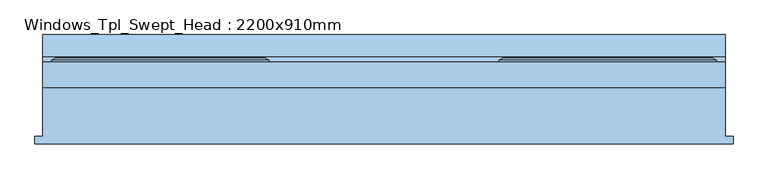
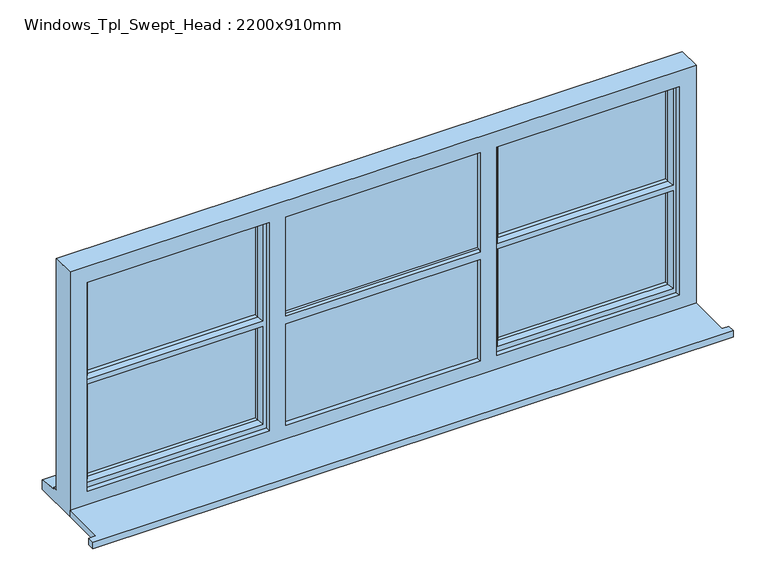
"""IFC4 building model written with IfcOpenShell, lengths in millimetres: window geometry, Windows_Tpl_Swept_Head : 2200x910mm."""

from ifc_helpers import new_model, si_unit, point, frame, frame_2d, origin, place, context, project, spatial, polyline, circle_curve, trimmed, segment, composite_curve, outline, extrude, faceted_brep, source, transform, mapped, element, save


def windows_tpl_swept_head_2200x910mm_9484ce63(model_context):
    return source(origin(), model_context, "Body", "SolidModel", [
        extrude(outline(polyline([(-1766.6666667, -161.5434322), (-1766.6666667, -136.5434322), (-1741.6666667, -136.5434322), (-1741.6666667, 20.4565678), (458.3333333, 20.4565678), (458.3333333, -136.5434322), (483.3333333, -136.5434322), (483.3333333, -161.5434322), (-1766.6666667, -161.5434322)])), frame((0.0, 0.0, 1200.0), z_axis=(0.0, 0.0, 1.0), x_axis=(1.0, 0.0, 0.0)), (0.0, 0.0, 1.0), 25.0),
        extrude(outline(composite_curve([segment(polyline([(2050.0, -300.0), (2050.0, -983.3333333), (1935.9532624, -983.3333333)]), True, "CONTINUOUS"), segment(trimmed(circle_curve(frame_2d((1325.0, -641.6666667)), 700.0), [point((1935.9532624, -983.3333333))], [point((1935.9532624, -300.0))], True, "CARTESIAN"), True, "CONTINUOUS"), segment(polyline([(1935.9532624, -300.0), (2050.0, -300.0)]), True, "CONTINUOUS")], self_intersect=False)), frame((0.0, 62.4565678, 0.0), z_axis=(0.0, 1.0, 0.0), x_axis=(0.0, 0.0, 1.0)), (0.0, 0.0, 1.0), 25.0),
        extrude(outline(composite_curve([segment(polyline([(2030.0, -220.0), (1957.8501446, -220.0)]), True, "CONTINUOUS"), segment(trimmed(circle_curve(frame_2d((1325.0, 79.1666667)), 700.0), [point((1957.8501446, -220.0))], [point((1957.8501446, 378.3333333))], True, "CARTESIAN"), True, "CONTINUOUS"), segment(polyline([(1957.8501446, 378.3333333), (2030.0, 378.3333333), (2030.0, -220.0)]), True, "CONTINUOUS")], self_intersect=False)), frame((0.0, 79.4565678, 0.0), z_axis=(0.0, 1.0, 0.0), x_axis=(0.0, 0.0, 1.0)), (0.0, 0.0, 1.0), 24.0),
        extrude(outline(composite_curve([segment(polyline([(2030.0, -1063.3333333), (2030.0, -1661.6666667), (1957.8501446, -1661.6666667)]), True, "CONTINUOUS"), segment(trimmed(circle_curve(frame_2d((1325.0, -1362.5)), 700.0), [point((1957.8501446, -1661.6666667))], [point((1957.8501446, -1063.3333333))], True, "CARTESIAN"), True, "CONTINUOUS"), segment(polyline([(1957.8501446, -1063.3333333), (2030.0, -1063.3333333)]), True, "CONTINUOUS")], self_intersect=False)), frame((0.0, 79.4565678, 0.0), z_axis=(0.0, 1.0, 0.0), x_axis=(0.0, 0.0, 1.0)), (0.0, 0.0, 1.0), 24.0),
        faceted_brep([(-270.0, 103.4565678, 2080.0), (-270.0, 109.2300705, 2080.0), (-270.0, 109.2300705, 1253.0), (-270.0, 103.4565678, 1253.0), (-260.0, 38.4565678, 2070.0), (-260.0, 103.4565678, 2070.0), (-260.0, 103.4565678, 1263.0), (-260.0, 38.4565678, 1263.0), (-220.0, 52.9494677, 2030.0), (-230.1480377, 38.4565678, 2040.1480377), (-230.1480377, 38.4565678, 1676.3519623), (-220.0, 52.9494677, 1686.5), (-230.1480377, 38.4565678, 1292.8519623), (-220.0, 52.9494677, 1303.0), (-220.0, 52.9494677, 1646.5), (-230.1480377, 38.4565678, 1656.6480377), (-220.0, 67.4565678, 2030.0), (-220.0, 67.4565678, 1686.5), (-220.0, 67.4565678, 1303.0), (-220.0, 67.4565678, 1646.5), (-230.0, 91.4565678, 1679.5), (-230.0, 91.4565678, 2040.0), (-230.0, 67.4565678, 2040.0), (-230.0, 67.4565678, 1679.5), (-230.0, 67.4565678, 1653.5), (-230.0, 67.4565678, 1293.0), (-230.0, 91.4565678, 1293.0), (-230.0, 91.4565678, 1653.5), (-220.0, 109.2300705, 2030.0), (-220.0, 91.4565678, 2030.0), (-220.0, 91.4565678, 1686.5), (-220.0, 109.2300705, 1686.5), (-220.0, 91.4565678, 1303.0), (-220.0, 109.2300705, 1303.0), (-220.0, 109.2300705, 1646.5), (-220.0, 91.4565678, 1646.5), (-237.4457548, 115.0035732, 2047.4457548), (-237.4457548, 115.0035732, 1669.0542452), (-237.4457548, 115.0035732, 1285.5542452), (-237.4457548, 115.0035732, 1663.9457548), (-259.2153903, 115.0035732, 2069.2153903), (-259.2153903, 115.0035732, 1263.7846097), (428.3333333, 109.2300705, 1253.0), (428.3333333, 103.4565678, 1253.0), (418.3333333, 103.4565678, 1263.0), (418.3333333, 38.4565678, 1263.0), (388.4813711, 38.4565678, 1292.8519623), (378.3333333, 52.9494677, 1303.0), (378.3333333, 67.4565678, 1303.0), (388.3333333, 67.4565678, 1293.0), (388.3333333, 91.4565678, 1293.0), (378.3333333, 91.4565678, 1303.0), (378.3333333, 109.2300705, 1303.0), (395.7790881, 115.0035732, 1285.5542452), (417.5487236, 115.0035732, 1263.7846097), (428.3333333, 109.2300705, 2080.0), (428.3333333, 103.4565678, 2080.0), (418.3333333, 103.4565678, 2070.0), (418.3333333, 38.4565678, 2070.0), (388.4813711, 38.4565678, 1656.6480377), (378.3333333, 52.9494677, 1646.5), (388.4813711, 38.4565678, 2040.1480377), (378.3333333, 52.9494677, 2030.0), (378.3333333, 52.9494677, 1686.5), (388.4813711, 38.4565678, 1676.3519623), (378.3333333, 67.4565678, 1646.5), (378.3333333, 67.4565678, 2030.0), (378.3333333, 67.4565678, 1686.5), (388.3333333, 91.4565678, 1653.5), (388.3333333, 67.4565678, 1653.5), (388.3333333, 67.4565678, 1679.5), (388.3333333, 67.4565678, 2040.0), (388.3333333, 91.4565678, 2040.0), (388.3333333, 91.4565678, 1679.5), (378.3333333, 91.4565678, 1646.5), (378.3333333, 109.2300705, 1646.5), (378.3333333, 91.4565678, 2030.0), (378.3333333, 109.2300705, 2030.0), (378.3333333, 109.2300705, 1686.5), (378.3333333, 91.4565678, 1686.5), (395.7790881, 115.0035732, 1663.9457548), (395.7790881, 115.0035732, 2047.4457548), (395.7790881, 115.0035732, 1669.0542452), (417.5487236, 115.0035732, 2069.2153903)], [[[0, 1, 2, 3]], [[4, 5, 6, 7]], [[8, 9, 10, 11]], [[12, 13, 14, 15]], [[16, 8, 11, 17]], [[13, 18, 19, 14]], [[20, 21, 22, 23]], [[24, 25, 26, 27]], [[28, 29, 30, 31]], [[32, 33, 34, 35]], [[36, 28, 31, 37]], [[33, 38, 39, 34]], [[2, 1, 40, 41]], [[3, 2, 42, 43]], [[7, 6, 44, 45]], [[13, 12, 46, 47]], [[18, 13, 47, 48]], [[26, 25, 49, 50]], [[33, 32, 51, 52]], [[38, 33, 52, 53]], [[2, 41, 54, 42]], [[43, 42, 55, 56]], [[45, 44, 57, 58]], [[47, 46, 59, 60]], [[61, 62, 63, 64]], [[48, 47, 60, 65]], [[62, 66, 67, 63]], [[68, 50, 49, 69]], [[70, 71, 72, 73]], [[52, 51, 74, 75]], [[76, 77, 78, 79]], [[53, 52, 75, 80]], [[77, 81, 82, 78]], [[42, 54, 83, 55]], [[1, 0, 56, 55]], [[0, 3, 43, 56], [6, 5, 57, 44]], [[5, 4, 58, 57]], [[4, 7, 45, 58], [46, 12, 15, 59], [61, 64, 10, 9]], [[9, 8, 62, 61]], [[8, 16, 66, 62]], [[49, 25, 24, 69], [18, 48, 65, 19]], [[22, 71, 70, 23], [66, 16, 17, 67]], [[22, 21, 72, 71]], [[26, 50, 68, 27], [32, 35, 74, 51]], [[72, 21, 20, 73], [76, 79, 30, 29]], [[29, 28, 77, 76]], [[28, 36, 81, 77]], [[41, 40, 83, 54], [36, 37, 82, 81], [38, 53, 80, 39]], [[40, 1, 55, 83]], [[82, 37, 31, 78]], [[30, 79, 78, 31]], [[73, 20, 23, 70]], [[11, 63, 67, 17]], [[10, 64, 63, 11]], [[59, 15, 14, 60]], [[60, 14, 19, 65]], [[27, 68, 69, 24]], [[74, 35, 34, 75]], [[39, 80, 75, 34]]]),
        faceted_brep([(-1013.3333333, 103.4565678, 2080.0), (-1013.3333333, 109.2300705, 2080.0), (-1711.6666667, 109.2300705, 2080.0), (-1711.6666667, 103.4565678, 2080.0), (-1023.3333333, 38.4565678, 2070.0), (-1023.3333333, 103.4565678, 2070.0), (-1701.6666667, 103.4565678, 2070.0), (-1701.6666667, 38.4565678, 2070.0), (-1063.3333333, 52.9494677, 2030.0), (-1053.1852956, 38.4565678, 2040.1480377), (-1671.8147044, 38.4565678, 2040.1480377), (-1661.6666667, 52.9494677, 2030.0), (-1661.6666667, 67.4565678, 2030.0), (-1063.3333333, 67.4565678, 2030.0), (-1053.3333333, 91.4565678, 2040.0), (-1053.3333333, 67.4565678, 2040.0), (-1671.6666667, 67.4565678, 2040.0), (-1671.6666667, 91.4565678, 2040.0), (-1063.3333333, 109.2300705, 2030.0), (-1063.3333333, 91.4565678, 2030.0), (-1661.6666667, 91.4565678, 2030.0), (-1661.6666667, 109.2300705, 2030.0), (-1679.1124215, 115.0035732, 2047.4457548), (-1045.8875785, 115.0035732, 2047.4457548), (-1024.117943, 115.0035732, 2069.2153903), (-1700.882057, 115.0035732, 2069.2153903), (-1711.6666667, 109.2300705, 1253.0), (-1711.6666667, 103.4565678, 1253.0), (-1701.6666667, 103.4565678, 1263.0), (-1701.6666667, 38.4565678, 1263.0), (-1671.8147044, 38.4565678, 1676.3519623), (-1661.6666667, 52.9494677, 1686.5), (-1671.8147044, 38.4565678, 1292.8519623), (-1661.6666667, 52.9494677, 1303.0), (-1661.6666667, 52.9494677, 1646.5), (-1671.8147044, 38.4565678, 1656.6480377), (-1661.6666667, 67.4565678, 1686.5), (-1661.6666667, 67.4565678, 1303.0), (-1661.6666667, 67.4565678, 1646.5), (-1671.6666667, 91.4565678, 1679.5), (-1671.6666667, 67.4565678, 1679.5), (-1671.6666667, 67.4565678, 1653.5), (-1671.6666667, 67.4565678, 1293.0), (-1671.6666667, 91.4565678, 1293.0), (-1671.6666667, 91.4565678, 1653.5), (-1661.6666667, 91.4565678, 1686.5), (-1661.6666667, 109.2300705, 1686.5), (-1661.6666667, 91.4565678, 1303.0), (-1661.6666667, 109.2300705, 1303.0), (-1661.6666667, 109.2300705, 1646.5), (-1661.6666667, 91.4565678, 1646.5), (-1679.1124215, 115.0035732, 1669.0542452), (-1679.1124215, 115.0035732, 1285.5542452), (-1679.1124215, 115.0035732, 1663.9457548), (-1700.882057, 115.0035732, 1263.7846097), (-1013.3333333, 109.2300705, 1253.0), (-1013.3333333, 103.4565678, 1253.0), (-1023.3333333, 103.4565678, 1263.0), (-1023.3333333, 38.4565678, 1263.0), (-1053.1852956, 38.4565678, 1676.3519623), (-1053.1852956, 38.4565678, 1656.6480377), (-1053.1852956, 38.4565678, 1292.8519623), (-1063.3333333, 52.9494677, 1303.0), (-1063.3333333, 67.4565678, 1303.0), (-1053.3333333, 67.4565678, 1679.5), (-1063.3333333, 67.4565678, 1686.5), (-1053.3333333, 67.4565678, 1293.0), (-1053.3333333, 67.4565678, 1653.5), (-1063.3333333, 67.4565678, 1646.5), (-1053.3333333, 91.4565678, 1293.0), (-1053.3333333, 91.4565678, 1679.5), (-1063.3333333, 91.4565678, 1686.5), (-1053.3333333, 91.4565678, 1653.5), (-1063.3333333, 91.4565678, 1646.5), (-1063.3333333, 91.4565678, 1303.0), (-1063.3333333, 109.2300705, 1303.0), (-1045.8875785, 115.0035732, 1285.5542452), (-1024.117943, 115.0035732, 1263.7846097), (-1045.8875785, 115.0035732, 1669.0542452), (-1045.8875785, 115.0035732, 1663.9457548), (-1063.3333333, 52.9494677, 1686.5), (-1063.3333333, 52.9494677, 1646.5), (-1063.3333333, 109.2300705, 1686.5), (-1063.3333333, 109.2300705, 1646.5)], [[[0, 1, 2, 3]], [[4, 5, 6, 7]], [[8, 9, 10, 11]], [[8, 11, 12, 13]], [[14, 15, 16, 17]], [[18, 19, 20, 21]], [[18, 21, 22, 23]], [[2, 1, 24, 25]], [[3, 2, 26, 27]], [[7, 6, 28, 29]], [[11, 10, 30, 31]], [[32, 33, 34, 35]], [[12, 11, 31, 36]], [[33, 37, 38, 34]], [[39, 17, 16, 40]], [[41, 42, 43, 44]], [[21, 20, 45, 46]], [[47, 48, 49, 50]], [[22, 21, 46, 51]], [[48, 52, 53, 49]], [[2, 25, 54, 26]], [[27, 26, 55, 56]], [[0, 3, 27, 56], [6, 5, 57, 28]], [[29, 28, 57, 58]], [[4, 7, 29, 58], [10, 9, 59, 30], [32, 35, 60, 61]], [[33, 32, 61, 62]], [[37, 33, 62, 63]], [[16, 15, 64, 40], [13, 12, 36, 65]], [[66, 42, 41, 67], [37, 63, 68, 38]], [[43, 42, 66, 69]], [[14, 17, 39, 70], [19, 71, 45, 20]], [[43, 69, 72, 44], [47, 50, 73, 74]], [[48, 47, 74, 75]], [[52, 48, 75, 76]], [[25, 24, 77, 54], [23, 22, 51, 78], [76, 79, 53, 52]], [[26, 54, 77, 55]], [[1, 0, 56, 55]], [[5, 4, 58, 57]], [[9, 8, 80, 59]], [[62, 61, 60, 81]], [[8, 13, 65, 80]], [[63, 62, 81, 68]], [[64, 15, 14, 70]], [[72, 69, 66, 67]], [[19, 18, 82, 71]], [[75, 74, 73, 83]], [[18, 23, 78, 82]], [[76, 75, 83, 79]], [[24, 1, 55, 77]], [[78, 51, 46, 82]], [[45, 71, 82, 46]], [[40, 64, 70, 39]], [[65, 36, 31, 80]], [[30, 59, 80, 31]], [[60, 35, 34, 81]], [[38, 68, 81, 34]], [[67, 41, 44, 72]], [[73, 50, 49, 83]], [[53, 79, 83, 49]]]),
        extrude(outline(polyline([(388.4813711, 67.4565678), (-230.0, 67.4565678), (-230.0, 91.4565678), (388.4813711, 91.4565678), (388.4813711, 67.4565678)])), frame((0.0, 0.0, 1293.0), z_axis=(0.0, 0.0, 1.0), x_axis=(1.0, 0.0, 0.0)), (0.0, 0.0, 1.0), 363.6480377),
        extrude(outline(polyline([(388.4813711, 67.4565678), (-230.0, 67.4565678), (-230.0, 91.4565678), (388.4813711, 91.4565678), (388.4813711, 67.4565678)])), frame((0.0, 0.0, 1676.3519623), z_axis=(0.0, 0.0, 1.0), x_axis=(1.0, 0.0, 0.0)), (0.0, 0.0, 1.0), 363.6480377),
        extrude(outline(polyline([(-993.3333333, 62.4565678), (-290.0, 62.4565678), (-290.0, 38.4565678), (-993.3333333, 38.4565678), (-993.3333333, 62.4565678)])), frame((0.0, 0.0, 1263.0), z_axis=(0.0, 0.0, 1.0), x_axis=(1.0, 0.0, 0.0)), (0.0, 0.0, 1.0), 390.5),
        extrude(outline(polyline([(-993.3333333, 62.4565678), (-290.0, 62.4565678), (-290.0, 38.4565678), (-993.3333333, 38.4565678), (-993.3333333, 62.4565678)])), frame((0.0, 0.0, 1679.5), z_axis=(0.0, 0.0, 1.0), x_axis=(1.0, 0.0, 0.0)), (0.0, 0.0, 1.0), 390.5),
        extrude(outline(polyline([(-1053.3333333, 67.4565678), (-1671.6666667, 67.4565678), (-1671.6666667, 91.4565678), (-1053.3333333, 91.4565678), (-1053.3333333, 67.4565678)])), frame((0.0, 0.0, 1676.3519623), z_axis=(0.0, 0.0, 1.0), x_axis=(1.0, 0.0, 0.0)), (0.0, 0.0, 1.0), 363.6480377),
        extrude(outline(polyline([(-1053.3333333, 67.4565678), (-1671.6666667, 67.4565678), (-1671.6666667, 91.4565678), (-1053.3333333, 91.4565678), (-1053.3333333, 67.4565678)])), frame((0.0, 0.0, 1293.0), z_axis=(0.0, 0.0, 1.0), x_axis=(1.0, 0.0, 0.0)), (0.0, 0.0, 1.0), 363.6480377),
        faceted_brep([(-983.3333333, 38.4565678, 2050.0), (-983.3333333, 20.4565678, 2050.0), (-983.3333333, 20.4565678, 1680.8390708), (-983.3333333, 28.5412125, 1686.5), (-983.3333333, 38.4565678, 1686.5), (-983.3333333, 20.4565678, 1275.0), (-983.3333333, 38.4565678, 1275.0), (-983.3333333, 38.4565678, 1646.5), (-983.3333333, 28.5412125, 1646.5), (-983.3333333, 20.4565678, 1652.1609292), (458.3333333, 20.4565678, 2110.0), (-1741.6666667, 20.4565678, 2110.0), (-1741.6666667, 20.4565678, 1200.0), (458.3333333, 20.4565678, 1200.0), (-1681.6666667, 20.4565678, 2050.0), (-1041.3333333, 20.4565678, 2050.0), (-1041.3333333, 20.4565678, 1275.0), (-1681.6666667, 20.4565678, 1275.0), (-242.0, 20.4565678, 2050.0), (398.3333333, 20.4565678, 2050.0), (398.3333333, 20.4565678, 1275.0), (-242.0, 20.4565678, 1275.0), (-300.0, 20.4565678, 2050.0), (-300.0, 20.4565678, 1680.8390708), (-300.0, 20.4565678, 1275.0), (-300.0, 20.4565678, 1652.1609292), (-1041.3333333, 38.4565678, 2050.0), (-1041.3333333, 38.4565678, 1275.0), (-1701.6666667, 38.4565678, 2070.0), (-1023.3333333, 38.4565678, 2070.0), (-1023.3333333, 38.4565678, 1263.0), (-1701.6666667, 38.4565678, 1263.0), (-1681.6666667, 38.4565678, 2050.0), (-1681.6666667, 38.4565678, 1275.0), (-993.3333333, 38.4565678, 2070.0), (-290.0, 38.4565678, 2070.0), (-290.0, 38.4565678, 1679.5), (-983.3333333, 38.4565678, 1679.5), (-983.3333333, 38.4565678, 1653.5), (-290.0, 38.4565678, 1653.5), (-290.0, 38.4565678, 1263.0), (-993.3333333, 38.4565678, 1263.0), (-300.0, 38.4565678, 2050.0), (-300.0, 38.4565678, 1686.5), (-300.0, 38.4565678, 1275.0), (-300.0, 38.4565678, 1646.5), (-260.0, 38.4565678, 2070.0), (418.3333333, 38.4565678, 2070.0), (418.3333333, 38.4565678, 1263.0), (-260.0, 38.4565678, 1263.0), (398.3333333, 38.4565678, 2050.0), (-242.0, 38.4565678, 2050.0), (-242.0, 38.4565678, 1275.0), (398.3333333, 38.4565678, 1275.0), (-1023.3333333, 103.4565678, 2070.0), (-1023.3333333, 103.4565678, 1263.0), (-1741.6666667, 103.4565678, 2110.0), (458.3333333, 103.4565678, 2110.0), (458.3333333, 103.4565678, 1251.0), (-1741.6666667, 103.4565678, 1251.0), (-1701.6666667, 103.4565678, 2070.0), (-1701.6666667, 103.4565678, 1263.0), (-983.3333333, 103.4565678, 2070.0), (-983.3333333, 103.4565678, 1263.0), (-300.0, 103.4565678, 1263.0), (-300.0, 103.4565678, 2070.0), (418.3333333, 103.4565678, 1263.0), (418.3333333, 103.4565678, 2070.0), (-260.0, 103.4565678, 2070.0), (-260.0, 103.4565678, 1263.0), (-983.3333333, 98.4565678, 2070.0), (-983.3333333, 98.4565678, 2050.0), (-983.3333333, 62.4565678, 2050.0), (-983.3333333, 62.4565678, 1686.5), (-983.3333333, 80.2300705, 1686.5), (-983.3333333, 86.0035732, 1669.0542452), (-983.3333333, 86.0035732, 1663.9457548), (-983.3333333, 80.2300705, 1646.5), (-983.3333333, 62.4565678, 1646.5), (-983.3333333, 62.4565678, 1275.0), (-983.3333333, 98.4565678, 1275.0), (-983.3333333, 98.4565678, 1263.0), (-290.0, 62.4565678, 1653.5), (-983.3333333, 62.4565678, 1653.5), (-983.3333333, 62.4565678, 1679.5), (-290.0, 62.4565678, 1679.5), (-290.0, 62.4565678, 2070.0), (-993.3333333, 62.4565678, 2070.0), (-993.3333333, 62.4565678, 1263.0), (-290.0, 62.4565678, 1263.0), (-300.0, 62.4565678, 2050.0), (-300.0, 62.4565678, 1686.5), (-300.0, 62.4565678, 1646.5), (-300.0, 62.4565678, 1275.0), (-1741.6666667, 118.4565678, 1249.68767), (-1741.6666667, 118.4565678, 1244.7449676), (-1741.6666667, 190.9565678, 1233.8088847), (-1741.6666667, 190.9565678, 1200.0), (-300.0, 98.4565678, 2070.0), (458.3333333, 190.9565678, 1200.0), (458.3333333, 190.9565678, 1233.8088847), (458.3333333, 118.4565678, 1244.7449676), (458.3333333, 118.4565678, 1249.68767), (-300.0, 98.4565678, 1263.0), (-300.0, 98.4565678, 1275.0), (-300.0, 80.2300705, 1646.5), (-300.0, 86.0035732, 1663.9457548), (-300.0, 86.0035732, 1669.0542452), (-300.0, 80.2300705, 1686.5), (-300.0, 98.4565678, 2050.0), (-300.0, 28.5412125, 1686.5), (-300.0, 28.5412125, 1646.5)], [[[0, 1, 2, 3, 4]], [[5, 6, 7, 8, 9]], [[10, 11, 12, 13], [14, 15, 16, 17], [18, 19, 20, 21], [1, 22, 23, 2], [24, 5, 9, 25]], [[15, 26, 27, 16]], [[28, 29, 30, 31], [26, 32, 33, 27]], [[34, 35, 36, 37, 38, 39, 40, 41], [42, 0, 4, 43], [6, 44, 45, 7]], [[46, 47, 48, 49], [50, 51, 52, 53]], [[54, 55, 30, 29]], [[56, 57, 58, 59], [55, 54, 60, 61], [62, 63, 64, 65], [66, 67, 68, 69]], [[63, 62, 70, 71, 72, 73, 74, 75, 76, 77, 78, 79, 80, 81]], [[82, 83, 84, 85, 86, 87, 88, 89], [73, 72, 90, 91], [92, 93, 79, 78]], [[88, 87, 34, 41]], [[11, 56, 59, 94, 95, 96, 97, 12]], [[61, 60, 28, 31]], [[32, 14, 17, 33]], [[11, 10, 57, 56]], [[62, 65, 98, 70]], [[87, 86, 35, 34]], [[28, 60, 54, 29]], [[67, 47, 46, 68]], [[1, 0, 42, 22]], [[14, 32, 26, 15]], [[50, 19, 18, 51]], [[57, 10, 13, 99, 100, 101, 102, 58]], [[67, 66, 48, 47]], [[19, 50, 53, 20]], [[82, 89, 40, 39]], [[35, 86, 85, 36]], [[65, 64, 103, 104, 93, 92, 105, 106, 107, 108, 91, 90, 109, 98]], [[69, 68, 46, 49]], [[51, 18, 21, 52]], [[22, 42, 43, 110, 23]], [[44, 24, 25, 111, 45]], [[99, 13, 12, 97]], [[100, 99, 97, 96]], [[101, 100, 96, 95]], [[102, 101, 95, 94]], [[58, 102, 94, 59]], [[55, 61, 31, 30]], [[64, 63, 81, 103]], [[66, 69, 49, 48]], [[89, 88, 41, 40]], [[17, 16, 27, 33]], [[21, 20, 53, 52]], [[44, 6, 5, 24]], [[83, 38, 37, 84]], [[75, 107, 106, 76]], [[76, 106, 105, 77]], [[92, 78, 77, 105]], [[38, 83, 82, 39]], [[7, 45, 111, 8]], [[25, 9, 8, 111]], [[2, 23, 110, 3]], [[43, 4, 3, 110]], [[84, 37, 36, 85]], [[73, 91, 108, 74]], [[107, 75, 74, 108]], [[79, 93, 104, 80]], [[80, 104, 103, 81]], [[109, 71, 70, 98]], [[90, 72, 71, 109]]]),
    ])


if __name__ == "__main__":
    model = new_model("IFC4")
    model_context = context("Model", 3, world=origin())
    ifc_project = project(units=[si_unit("LENGTHUNIT", "METRE", prefix="MILLI")], contexts=[model_context])
    site = spatial("IfcSite", under=ifc_project)
    building = spatial("IfcBuilding", under=site)
    placement = place(None, origin())
    windows_tpl_swept_head_2200x910mm_shape = windows_tpl_swept_head_2200x910mm_9484ce63(model_context)
    element("IfcWindow", 1, ObjectType="Windows_Tpl_Swept_Head : 2200x910mm", at=placement, inside=building, context=model_context, shape_type="MappedRepresentation", body=[
        mapped(windows_tpl_swept_head_2200x910mm_shape, transform((0.0, 0.0, 0.0), x_axis=(1.0, 0.0, 0.0), y_axis=(0.0, 1.0, 0.0), z_axis=(0.0, 0.0, 1.0))),
    ])
    save(model, "model.ifc")

# Revit data of these elements
# Type "Windows_Tpl_Swept_Head : 2200x910mm"
#   Type Mark = "56"
#   Operation = "TriplePanelVertical"
#   Construction Type Id = "GSP4R"
#   Manufacturer = "Revit"
#   Keynote = "L10"
#   Analytic Construction = "1/8 in Pilkington single glazing"
#   Wrap Layers (Ext) from Ext = 102.5 mm
#   Wrap Layers (Int) from Ext = 177.5 mm
#   Window Board Projection = 25 mm
#   Window Board Extension = 25 mm
#   Visual Light Transmittance = 0.9
#   Solar Heat Gain Coefficient = 0.78
#   Rough Width = 2200 mm
#   Rough Height = 910 mm
#   Radius - Swept Head = 700 mm
#   Height = 910 mm
#   Width = 2200 mm
#   Heat Transfer Coefficient (U) = 3.6886 W/(m²·K)
#   Glazing Thickness = 24 mm
#   FrameOffset - External = 50 mm
#   Frame Depth = 65 mm
#   Default Head Height = 2110 mm
#   Cill Depth = 87.5 mm
#   Cavity Closer Width = 50 mm
#   Cavity Closer Offset from Ext = 102.5 mm
#   Cavity Closer Depth = 85 mm
#   Vis - Cavity Closers = yes
#   Material Trim = Window Frame
#   Material Glass = Glass
#   Material Frame = Window Frame
#   Wall Closure = (empty or 0)
# Element 1 (IfcWindow, "Windows_Tpl_Swept_Head : 2200x910mm")
#   Materials on its faces: "Window Frame", "Glass"
# Materials
#   "Window Frame": class "Miscellaneous", colour RGB 249 249 249, transparency 0, Keynote = "L10", Cost = 0
#   "Glass": class "Glass", colour RGB 0 128 192, transparency 0.9, Description = "Soda Lime Glass", Cost = 0
